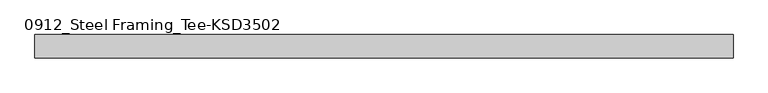
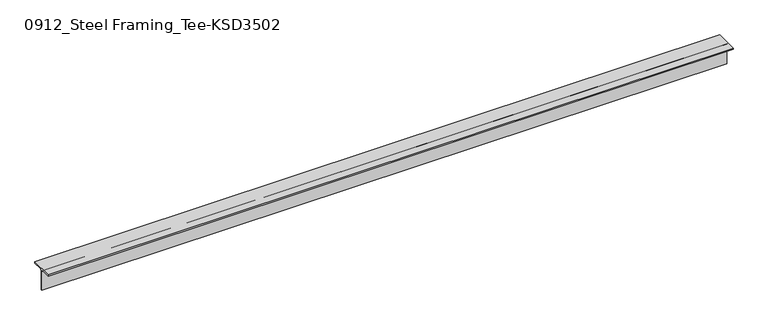
"""IFC4 building model written with IfcOpenShell, lengths in millimetres: member geometry, 0912_Steel Framing_Tee-KSD3502 : H_SB_ASB_CT-150x150x6.5x9."""

from ifc_helpers import new_model, si_unit, point, frame, frame_2d, origin, place, context, project, spatial, polyline, circle_curve, trimmed, segment, composite_curve, outline, extrude, source, transform, mapped, element, save


def member_0912_steel_framing_tee_ksd3502_c2bbe445(model_context):
    return source(origin(), model_context, "Body", "SweptSolid", [
        extrude(outline(composite_curve([segment(polyline([(-75.0, 75.0), (75.0, 75.0), (75.0, 66.0), (16.25, 66.0)]), True, "CONTINUOUS"), segment(trimmed(circle_curve(frame_2d((16.25, 53.0)), 13.0), [point((16.25, 66.0))], [point((3.25, 53.0))], True, "CARTESIAN"), True, "CONTINUOUS"), segment(polyline([(3.25, 53.0), (3.25, -75.0), (-3.25, -75.0), (-3.25, 53.0)]), True, "CONTINUOUS"), segment(trimmed(circle_curve(frame_2d((-16.25, 53.0)), 13.0), [point((-3.25, 53.0))], [point((-16.25, 66.0))], True, "CARTESIAN"), True, "CONTINUOUS"), segment(polyline([(-16.25, 66.0), (-75.0, 66.0), (-75.0, 75.0)]), True, "CONTINUOUS")], self_intersect=False)), frame((-2233.2, 0.0, 0.0), z_axis=(1.0, 0.0, 0.0), x_axis=(0.0, 1.0, 0.0)), (0.0, 0.0, 1.0), 4448.4),
    ])


if __name__ == "__main__":
    model = new_model("IFC4")
    model_context = context("Model", 3, world=origin())
    ifc_project = project(units=[si_unit("LENGTHUNIT", "METRE", prefix="MILLI")], contexts=[model_context])
    site = spatial("IfcSite", under=ifc_project)
    building = spatial("IfcBuilding", under=site)
    placement = place(None, origin())
    member_0912_steel_framing_tee_ksd3502_shape = member_0912_steel_framing_tee_ksd3502_c2bbe445(model_context)
    element("IfcMember", 1, ObjectType="0912_Steel Framing_Tee-KSD3502 : H_SB_ASB_CT-150x150x6.5x9", at=placement, inside=building, context=model_context, shape_type="MappedRepresentation", body=[
        mapped(member_0912_steel_framing_tee_ksd3502_shape, transform((0.0, 0.0, 0.0), x_axis=(1.0, 0.0, 0.0), y_axis=(0.0, 1.0, 0.0), z_axis=(0.0, 0.0, 1.0))),
    ])
    save(model, "model.ifc")

# Revit data of these elements
# Type "0912_Steel Framing_Tee-KSD3502 : H_SB_ASB_CT-150x150x6.5x9"
#   H_WM Code_1 = "S01AA003-00001 | Main Steel Structure Fabrication Work | Shelter/Building | Light Steel - Standard (30KG/M>Weight) | Material: (   )"
#   H_WM Code_2 = "S03AA029-00001 | Main Steel Structure Erection Work | Shelter/Building | Light Steel (30KG/M>Weight) | Material: (   )"
#   H_WM Code_3 = "S01AA010-00001 | Main Steel Structure Fabrication Work | Shelter/Building | Steel Painting/Coating | for Non-Fireproofed Steel Surface, Surface Preparation, Primer, Second & Final Coat | Material: (   )"
#   H_Q'ty Cal Type Tag = "SB-Q2"
#   Width = 15.0 cm
#   Web Thickness = 0.65 cm
#   Web Fillet = 1.3 cm
#   Section Area = 23.39 cm²
#   Perimeter = 0.60 m²/m
#   Nominal Weight = 18.40 kgf/m
#   Height = 15.0 cm
#   Flange Thickness = 0.9 cm
#   Centroid Vertical = 7.5 cm
#   Centroid Horizontal = 7.5 cm
#   Length [instance default] = 1.5000 m
#   Structural Material [instance default] = Steel, 45-345
#   Warping Constant = (empty or 0)
#   Torsional Moment of Inertia = 0
#   Section Name Key = ""
#   Plastic Modulus weak axis = 0
#   Plastic Modulus strong axis = 0
#   Moment of Inertia weak axis = 0
#   Moment of Inertia strong axis = 0
#   Elastic Modulus weak axis = 0
#   Elastic Modulus strong axis = 0
#   Bolt Spacing = 0
#   Assembly Code = ""
# Element 1 (IfcMember, "0912_Steel Framing_Tee-KSD3502 : H_SB_ASB_CT-150x150x6.5x9")
#   Structural Material = none
# Materials
#   "Steel, 45-345": class "Metal", colour RGB 189 187 185, transparency 0, Description = "Steel 345 MPa", Cost = 0
